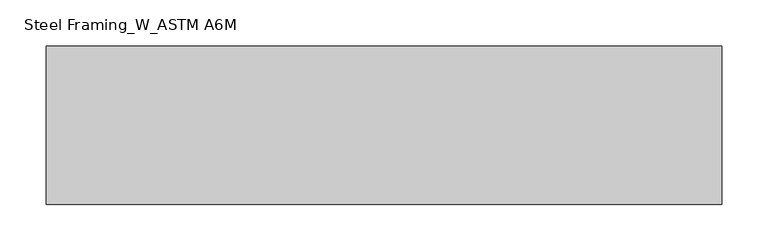
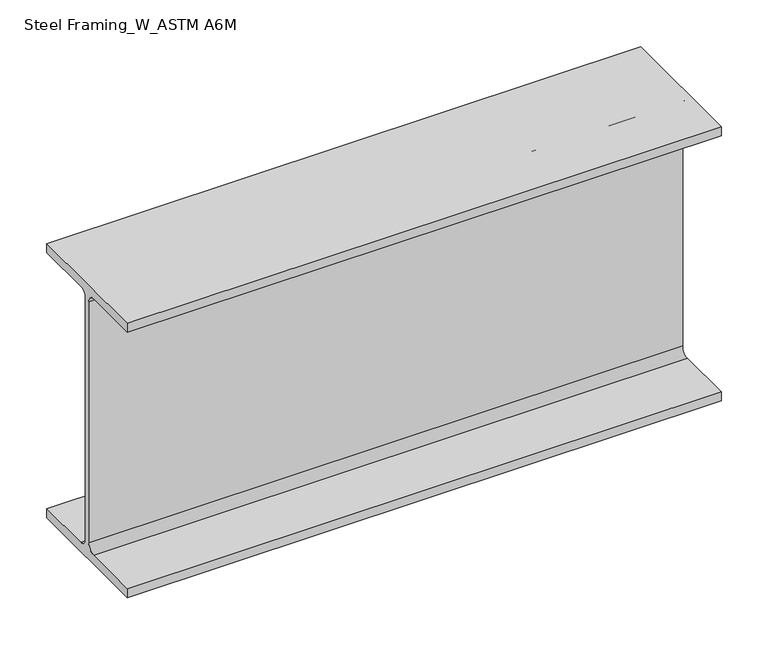
"""IFC4 building model written with IfcOpenShell, lengths in millimetres: beam geometry, Steel Framing_W_ASTM A6M : H_SB_AR_S02_W360x51_RG1."""

from ifc_helpers import new_model, si_unit, point, frame, frame_2d, origin, place, context, project, spatial, polyline, circle_curve, trimmed, segment, composite_curve, outline, extrude, source, transform, mapped, element, save


def steel_framing_w_astm_a6m_53a89d7e(model_context):
    return source(origin(), model_context, "Body", "SweptSolid", [
        extrude(outline(composite_curve([segment(polyline([(85.5, -166.4), (85.5, -178.0), (-85.5, -178.0), (-85.5, -166.4), (-13.72, -166.4)]), True, "CONTINUOUS"), segment(trimmed(circle_curve(frame_2d((-13.72, -156.3)), 10.1), [point((-13.72, -166.4))], [point((-3.62, -156.3))], True, "CARTESIAN"), True, "CONTINUOUS"), segment(polyline([(-3.62, -156.3), (-3.62, 156.3)]), True, "CONTINUOUS"), segment(trimmed(circle_curve(frame_2d((-13.72, 156.3)), 10.1), [point((-3.62, 156.3))], [point((-13.72, 166.4))], True, "CARTESIAN"), True, "CONTINUOUS"), segment(polyline([(-13.72, 166.4), (-85.5, 166.4), (-85.5, 178.0), (85.5, 178.0), (85.5, 166.4), (13.72, 166.4)]), True, "CONTINUOUS"), segment(trimmed(circle_curve(frame_2d((13.72, 156.3)), 10.1), [point((13.72, 166.4))], [point((3.62, 156.3))], True, "CARTESIAN"), True, "CONTINUOUS"), segment(polyline([(3.62, 156.3), (3.62, -156.3)]), True, "CONTINUOUS"), segment(trimmed(circle_curve(frame_2d((13.72, -156.3)), 10.1), [point((3.62, -156.3))], [point((13.72, -166.4))], True, "CARTESIAN"), True, "CONTINUOUS"), segment(polyline([(13.72, -166.4), (85.5, -166.4)]), True, "CONTINUOUS")], self_intersect=False)), frame((-480.8, 0.0, 0.0), z_axis=(1.0, 0.0, 0.0), x_axis=(0.0, 1.0, 0.0)), (0.0, 0.0, 1.0), 729.3),
    ])


if __name__ == "__main__":
    model = new_model("IFC4")
    model_context = context("Model", 3, world=origin())
    ifc_project = project(units=[si_unit("LENGTHUNIT", "METRE", prefix="MILLI")], contexts=[model_context])
    site = spatial("IfcSite", under=ifc_project)
    building = spatial("IfcBuilding", under=site)
    placement = place(None, origin())
    steel_framing_w_astm_a6m_shape = steel_framing_w_astm_a6m_53a89d7e(model_context)
    element("IfcBeam", 1, ObjectType="Steel Framing_W_ASTM A6M : H_SB_AR_S02_W360x51_RG1", at=placement, inside=building, context=model_context, shape_type="MappedRepresentation", body=[
        mapped(steel_framing_w_astm_a6m_shape, transform((0.0, 0.0, 0.0), x_axis=(1.0, 0.0, 0.0), y_axis=(0.0, 1.0, 0.0), z_axis=(0.0, 0.0, 1.0))),
    ])
    save(model, "model.ifc")

# Revit data of these elements
# Type "Steel Framing_W_ASTM A6M : H_SB_AR_S02_W360x51_RG1"
#   Type Mark = "RG1"
#   Section Name Key = "W14x34"
#   Width = 17.1 cm
#   Web Thickness = 0.724 cm
#   Web Fillet = 1.01 cm
#   Warping Constant = 287000.0 cm⁶
#   Torsional Moment of Inertia = 23.70 cm⁴
#   Section Area = 64.5 cm²
#   Plastic Modulus weak axis = 174.0 cm³
#   Plastic Modulus strong axis = 895.0 cm³
#   Perimeter = 1.36 m²/m
#   Nominal Weight = 51.00 kgf/m
#   Moment of Inertia weak axis = 970.00 cm⁴
#   Moment of Inertia strong axis = 14200.00 cm⁴
#   Height = 35.6 cm
#   Flange Thickness = 1.16 cm
#   Elastic Modulus weak axis = 113.0 cm³
#   Elastic Modulus strong axis = 796.0 cm³
#   Centroid Vertical = 17.8 cm
#   Centroid Horizontal = 8.55 cm
#   Length [instance default] = 1500 mm
#   Structural Material [instance default] = Steel, 45-345
#   Bolt Spacing = 0
#   Assembly Code = ""
# Element 1 (IfcBeam, "Steel Framing_W_ASTM A6M : H_SB_AR_S02_W360x51_RG1")
#   Materials on its faces: "Steel, 45-345"
# Materials
#   "Steel, 45-345": class "Metal", colour RGB 189 187 185, transparency 0, Description = "Steel 345 MPa", Cost = 0
